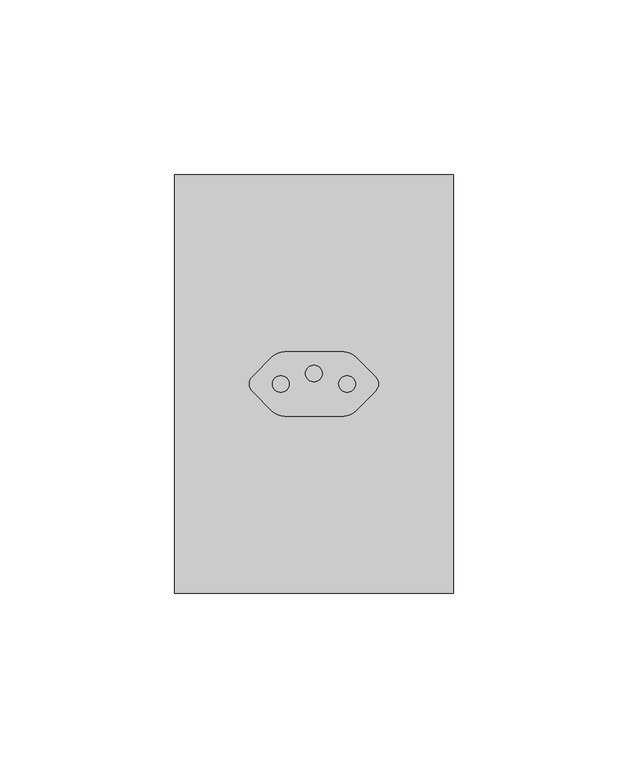
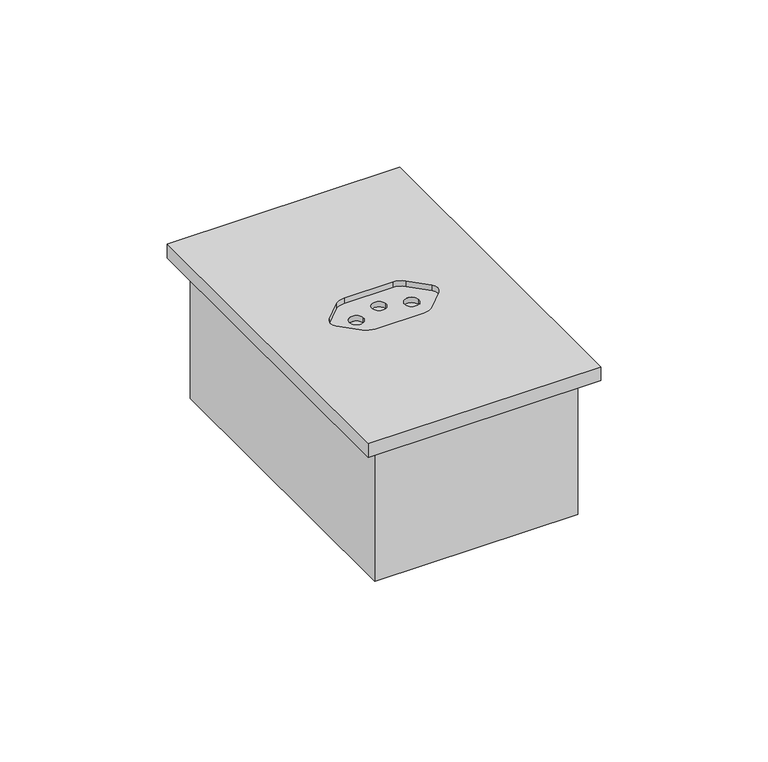
"""IFC4 building model written with IfcOpenShell, lengths in millimetres: proxy geometry, CAIXA VERTICE V7 : Tomada 20A 1s."""

from ifc_helpers import new_model, si_unit, frame, origin, place, context, project, spatial, polyline, circle_curve, faceted_brep, source, transform, mapped, element, save
from ifc_brep_helpers import plane_surface, revolved_surface, advanced_brep


def electrical_fixtures_f81dfd5c(model_context):
    return source(origin(), model_context, "Body", "SolidModel", [
        faceted_brep([(33.0, 2197.0, -48.0), (33.0, 2303.0, -48.0), (-33.0, 2303.0, -48.0), (-33.0, 2197.0, -48.0), (35.0, 2305.0, -50.0), (35.0, 2195.0, -50.0), (-35.0, 2195.0, -50.0), (-35.0, 2305.0, -50.0), (-35.0, 2305.0, 0.0), (35.0, 2305.0, 0.0), (-35.0, 2195.0, 0.0), (35.0, 2195.0, 0.0), (33.0, 2303.0, 0.0), (33.0, 2197.0, 0.0), (-33.0, 2197.0, 0.0), (-33.0, 2303.0, 0.0)], [[[0, 1, 2, 3]], [[4, 5, 6, 7]], [[4, 7, 8, 9]], [[8, 7, 6, 10]], [[10, 6, 5, 11]], [[11, 5, 4, 9]], [[9, 8, 10, 11], [12, 13, 14, 15]], [[13, 12, 1, 0]], [[14, 13, 0, 3]], [[15, 14, 3, 2]], [[12, 15, 2, 1]]]),
        advanced_brep(
        [(40.0, 2310.0, 5.0), (-40.0, 2310.0, 5.0), (-40.0, 2190.0, 5.0), (40.0, 2190.0, 5.0), (8.4215729, 2240.75, 5.0), (-8.4215729, 2240.75, 5.0), (-11.9571068, 2242.2144661, 5.0), (-17.6213203, 2247.8786797, 5.0), (-17.6213203, 2252.1213203, 5.0), (-11.9571068, 2257.7855339, 5.0), (-8.4215729, 2259.25, 5.0), (8.4215729, 2259.25, 5.0), (11.9571068, 2257.7855339, 5.0), (17.6213203, 2252.1213203, 5.0), (17.6213203, 2247.8786797, 5.0), (11.9571068, 2242.2144661, 5.0), (-40.0, 2310.0, 0.0), (40.0, 2310.0, 0.0), (40.0, 2190.0, 0.0), (-40.0, 2190.0, 0.0), (8.4215729, 2240.75, 3.0), (11.9571068, 2242.2144661, 3.0), (17.6213203, 2247.8786797, 3.0), (17.6213203, 2252.1213203, 3.0), (11.9571068, 2257.7855339, 3.0), (8.4215729, 2259.25, 3.0), (-8.4215729, 2259.25, 3.0), (-11.9571068, 2257.7855339, 3.0), (-17.6213203, 2252.1213203, 3.0), (-17.6213203, 2247.8786797, 3.0), (-11.9571068, 2242.2144661, 3.0), (-8.4215729, 2240.75, 3.0), (-7.1, 2250.0, 3.0), (-11.9, 2250.0, 3.0), (11.9, 2250.0, 3.0), (7.1, 2250.0, 3.0), (2.4, 2253.0, 3.0), (-2.4, 2253.0, 3.0), (-11.9, 2250.0, 1.0), (-7.1, 2250.0, 1.0), (7.1, 2250.0, 1.0), (11.9, 2250.0, 1.0), (-2.4, 2253.0, 1.0), (2.4, 2253.0, 1.0)],
        [
            (0, 1),
            (1, 2),
            (2, 3),
            (3, 0),
            (4, 5),
            (5, 6, circle_curve(frame((-8.4215729, 2245.75, 5.0), z_axis=(0.0, 0.0, -1.0), x_axis=(-1.0, 0.0, 0.0)), 5.0)),
            (6, 7),
            (7, 8, circle_curve(frame((-15.5, 2250.0, 5.0), z_axis=(0.0, 0.0, -1.0), x_axis=(-1.0, 0.0, 0.0)), 3.0)),
            (8, 9),
            (9, 10, circle_curve(frame((-8.4215729, 2254.25, 5.0), z_axis=(0.0, 0.0, -1.0), x_axis=(-1.0, 0.0, 0.0)), 5.0)),
            (10, 11),
            (11, 12, circle_curve(frame((8.4215729, 2254.25, 5.0), z_axis=(0.0, 0.0, -1.0), x_axis=(-1.0, 0.0, 0.0)), 5.0)),
            (12, 13),
            (13, 14, circle_curve(frame((15.5, 2250.0, 5.0), z_axis=(0.0, 0.0, -1.0), x_axis=(-1.0, 0.0, 0.0)), 3.0)),
            (14, 15),
            (15, 4, circle_curve(frame((8.4215729, 2245.75, 5.0), z_axis=(0.0, 0.0, -1.0), x_axis=(-1.0, 0.0, 0.0)), 5.0)),
            (16, 17),
            (17, 18),
            (18, 19),
            (19, 16),
            (0, 17),
            (16, 1),
            (19, 2),
            (18, 3),
            (20, 21, circle_curve(frame((8.4215729, 2245.75, 3.0), z_axis=(0.0, 0.0, 1.0), x_axis=(-1.0, 0.0, 0.0)), 5.0)),
            (21, 22),
            (22, 23, circle_curve(frame((15.5, 2250.0, 3.0), z_axis=(0.0, 0.0, 1.0), x_axis=(-1.0, 0.0, 0.0)), 3.0)),
            (23, 24),
            (24, 25, circle_curve(frame((8.4215729, 2254.25, 3.0), z_axis=(0.0, 0.0, 1.0), x_axis=(-1.0, 0.0, 0.0)), 5.0)),
            (25, 26),
            (26, 27, circle_curve(frame((-8.4215729, 2254.25, 3.0), z_axis=(0.0, 0.0, 1.0), x_axis=(-1.0, 0.0, 0.0)), 5.0)),
            (27, 28),
            (28, 29, circle_curve(frame((-15.5, 2250.0, 3.0), z_axis=(0.0, 0.0, 1.0), x_axis=(-1.0, 0.0, 0.0)), 3.0)),
            (29, 30),
            (30, 31, circle_curve(frame((-8.4215729, 2245.75, 3.0), z_axis=(0.0, 0.0, 1.0), x_axis=(-1.0, 0.0, 0.0)), 5.0)),
            (31, 20),
            (32, 33, circle_curve(frame((-9.5, 2250.0, 3.0), z_axis=(0.0, 0.0, -1.0), x_axis=(1.0, 2.301812013077709e-12, 0.0)), 2.4)),
            (33, 32, circle_curve(frame((-9.5, 2250.0, 3.0), z_axis=(0.0, 0.0, -1.0), x_axis=(1.0, 2.301812013077709e-12, 0.0)), 2.4)),
            (34, 35, circle_curve(frame((9.5, 2250.0, 3.0), z_axis=(0.0, 0.0, -1.0), x_axis=(1.0, 2.301812013077709e-12, 0.0)), 2.4)),
            (35, 34, circle_curve(frame((9.5, 2250.0, 3.0), z_axis=(0.0, 0.0, -1.0), x_axis=(1.0, 2.301812013077709e-12, 0.0)), 2.4)),
            (36, 37, circle_curve(frame((0.0, 2253.0, 3.0), z_axis=(0.0, 0.0, -1.0), x_axis=(1.0, 2.301812013077709e-12, 0.0)), 2.4)),
            (37, 36, circle_curve(frame((0.0, 2253.0, 3.0), z_axis=(0.0, 0.0, -1.0), x_axis=(1.0, 2.301812013077709e-12, 0.0)), 2.4)),
            (31, 5),
            (4, 20),
            (30, 6),
            (29, 7),
            (28, 8),
            (27, 9),
            (26, 10),
            (25, 11),
            (24, 12),
            (23, 13),
            (22, 14),
            (21, 15),
            (38, 39, circle_curve(frame((-9.5, 2250.0, 1.0), z_axis=(0.0, 0.0, 1.0), x_axis=(1.0, 2.301812013077709e-12, 0.0)), 2.4)),
            (39, 38, circle_curve(frame((-9.5, 2250.0, 1.0), z_axis=(0.0, 0.0, 1.0), x_axis=(1.0, 2.301812013077709e-12, 0.0)), 2.4)),
            (40, 41, circle_curve(frame((9.5, 2250.0, 1.0), z_axis=(0.0, 0.0, 1.0), x_axis=(1.0, 2.301812013077709e-12, 0.0)), 2.4)),
            (41, 40, circle_curve(frame((9.5, 2250.0, 1.0), z_axis=(0.0, 0.0, 1.0), x_axis=(1.0, 2.301812013077709e-12, 0.0)), 2.4)),
            (42, 43, circle_curve(frame((0.0, 2253.0, 1.0), z_axis=(0.0, 0.0, 1.0), x_axis=(1.0, 2.301812013077709e-12, 0.0)), 2.4)),
            (43, 42, circle_curve(frame((0.0, 2253.0, 1.0), z_axis=(0.0, 0.0, 1.0), x_axis=(1.0, 2.301812013077709e-12, 0.0)), 2.4)),
            (32, 39),
            (38, 33),
            (34, 41),
            (40, 35),
            (36, 43),
            (42, 37),
        ],
        [
            plane_surface(frame((-60.0, 2310.0, 5.0), z_axis=(0.0, 0.0, 1.0), x_axis=(-1.0, 0.0, 0.0))),
            plane_surface(frame((-60.0, 2310.0, 0.0), z_axis=(0.0, 0.0, -1.0), x_axis=(1.0, 0.0, 0.0))),
            plane_surface(frame((40.0, 2310.0, 5.0), z_axis=(0.0, 1.0, 0.0), x_axis=(0.0, 0.0, -1.0))),
            plane_surface(frame((-40.0, 2310.0, 5.0), z_axis=(-1.0, 0.0, 0.0), x_axis=(0.0, 0.0, -1.0))),
            plane_surface(frame((-40.0, 2190.0, 5.0), z_axis=(0.0, -1.0, 0.0), x_axis=(0.0, 0.0, -1.0))),
            plane_surface(frame((40.0, 2190.0, 5.0), z_axis=(1.0, 0.0, 0.0), x_axis=(0.0, 0.0, -1.0))),
            plane_surface(frame((3.4215729, 2245.75, 3.0), z_axis=(0.0, 0.0, 1.0), x_axis=(0.0, 1.0, 0.0))),
            plane_surface(frame((-8.4215729, 2240.75, 5.0), z_axis=(0.0, 1.0, 0.0), x_axis=(0.0, 0.0, -1.0))),
            revolved_surface(polyline([(-13.4215729, 2245.75, 5.0), (-13.4215729, 2245.75, 3.0)]), (-8.4215729, 2245.75, 3.0), (0.0, 0.0, 1.0)),
            plane_surface(frame((-17.6213203, 2247.8786797, 5.0), z_axis=(0.7071067811865045, 0.7071067811865905, 0.0), x_axis=(0.0, 0.0, -1.0))),
            revolved_surface(polyline([(-18.5, 2250.0, 5.0), (-18.5, 2250.0, 3.0)]), (-15.5, 2250.0, 3.0), (0.0, 0.0, 1.0)),
            plane_surface(frame((-11.9571068, 2257.7855339, 5.0), z_axis=(0.7071067811865515, -0.7071067811865437, 0.0), x_axis=(0.0, 0.0, -1.0))),
            revolved_surface(polyline([(-13.4215729, 2254.25, 5.0), (-13.4215729, 2254.25, 3.0)]), (-8.4215729, 2254.25, 3.0), (0.0, 0.0, 1.0)),
            plane_surface(frame((8.4215729, 2259.25, 5.0), z_axis=(0.0, -1.0, 0.0), x_axis=(0.0, 0.0, -1.0))),
            revolved_surface(polyline([(3.4215728999999993, 2254.25, 5.0), (3.4215728999999993, 2254.25, 3.0)]), (8.4215729, 2254.25, 3.0), (0.0, 0.0, 1.0)),
            plane_surface(frame((17.6213203, 2252.1213203, 5.0), z_axis=(-0.7071067811865307, -0.7071067811865643, 0.0), x_axis=(0.0, 0.0, -1.0))),
            revolved_surface(polyline([(12.5, 2250.0, 5.0), (12.5, 2250.0, 3.0)]), (15.5, 2250.0, 3.0), (0.0, 0.0, 1.0)),
            plane_surface(frame((11.9571068, 2242.2144661, 5.0), z_axis=(-0.7071067811865893, 0.7071067811865058, 0.0), x_axis=(0.0, 0.0, -1.0))),
            revolved_surface(polyline([(3.4215728999999993, 2245.75, 5.0), (3.4215728999999993, 2245.75, 3.0)]), (8.4215729, 2245.75, 3.0), (0.0, 0.0, 1.0)),
            plane_surface(frame((-7.1, 2250.0, 1.0), z_axis=(0.0, 0.0, 1.0), x_axis=(2.301812013077709e-12, -1.0, 0.0))),
            revolved_surface(polyline([(-7.1, 2250.0000000000055, 3.0), (-7.1, 2250.0000000000055, 1.0)]), (-9.5, 2250.0, 1.0), (0.0, 0.0, 1.0)),
            revolved_surface(polyline([(11.9, 2250.0000000000055, 3.0), (11.9, 2250.0000000000055, 1.0)]), (9.5, 2250.0, 5.0), (0.0, 0.0, 1.0)),
            revolved_surface(polyline([(2.4, 2253.0000000000055, 3.0), (2.4, 2253.0000000000055, 1.0)]), (0.0, 2253.0, 5.0), (0.0, 0.0, 1.0)),
        ],
        [
            (0, [[1, 2, 3, 4], [5, 6, 7, 8, 9, 10, 11, 12, 13, 14, 15, 16]]),
            (1, [[17, 18, 19, 20]]),
            (2, [[-1, 21, -17, 22]]),
            (3, [[-2, -22, -20, 23]]),
            (4, [[-3, -23, -19, 24]]),
            (5, [[-4, -24, -18, -21]]),
            (6, [[25, 26, 27, 28, 29, 30, 31, 32, 33, 34, 35, 36], [37, 38], [39, 40], [41, 42]]),
            (7, [[-36, 43, -5, 44]]),
            (8, [[-35, 45, -6, -43]]),
            (9, [[-34, 46, -7, -45]]),
            (10, [[-33, 47, -8, -46]]),
            (11, [[-32, 48, -9, -47]]),
            (12, [[-31, 49, -10, -48]]),
            (13, [[-30, 50, -11, -49]]),
            (14, [[-29, 51, -12, -50]]),
            (15, [[-28, 52, -13, -51]]),
            (16, [[-27, 53, -14, -52]]),
            (17, [[-26, 54, -15, -53]]),
            (18, [[-25, -44, -16, -54]]),
            (19, [[55, 56]]),
            (19, [[57, 58]]),
            (19, [[59, 60]]),
            (20, [[-37, 61, -55, 62]]),
            (20, [[-38, -62, -56, -61]]),
            (21, [[-39, 63, -57, 64]]),
            (21, [[-40, -64, -58, -63]]),
            (22, [[-41, 65, -59, 66]]),
            (22, [[-42, -66, -60, -65]]),
        ],
    ),
    ])


if __name__ == "__main__":
    model = new_model("IFC4")
    model_context = context("Model", 3, world=origin())
    ifc_project = project(units=[si_unit("LENGTHUNIT", "METRE", prefix="MILLI")], contexts=[model_context])
    site = spatial("IfcSite", under=ifc_project)
    building = spatial("IfcBuilding", under=site)
    placement = place(None, origin())
    electrical_fixtures_shape = electrical_fixtures_f81dfd5c(model_context)
    element("IfcBuildingElementProxy", 1, Name="CAIXA VERTICE V7 : Tomada 20A 1s", ObjectType="CAIXA VERTICE V7 : Tomada 20A 1s", at=placement, inside=building, context=model_context, shape_type="MappedRepresentation", body=[
        mapped(electrical_fixtures_shape, transform((0.0, 0.0, 0.0), x_axis=(1.0, 0.0, 0.0), y_axis=(0.0, 1.0, 0.0), z_axis=(0.0, 0.0, 1.0))),
    ])
    save(model, "model.ifc")

# Revit data of these elements
# Type "CAIXA VERTICE V7 : Tomada 20A 1s"
#   URL = "www.facebook.com/verticetreinamentos"
#   SEÇÃO [instance default] = ""
#   Rotação [instance default] = 0.00°
#   LARGURA DA TAMPA = 0.08 m
#   BORDA = 0.01 m
#   ALTURA DE INSTALAÇÃO [instance default] = 1.10 m
#   Distância Anotação [instance default] = 0.0015 m
#   ALTURA DA TAMPA = 0.12 m
#   Vertical [instance default] = yes
#   VER SEÇÃO [instance default] = no
#   SHADE ESQ [instance default] = no
#   SHADE DIR [instance default] = yes
#   HORIZONTAL [instance default] = no
#   ANDAR COM A LEGENDA [instance default] = 0
#   Material Tampa [instance default] = Plástico, branco opaco
#   Caixa = element 1798517
#   Anotação = element 1798531
#   Default Elevation = 0
# Element 1 (IfcBuildingElementProxy, "CAIXA VERTICE V7 : Tomada 20A 1s")
#   ALTURA DE INSTALAÇÃO = 2.25 m
#   SHADE ESQ = yes
#   Materials on its faces: "Plástico, branco opaco"
# Materials
#   "Plástico, branco opaco": class "Plástico", colour RGB 120 120 120, transparency 0, Description = "Plastic, generic, opaque white", Cost = 0
